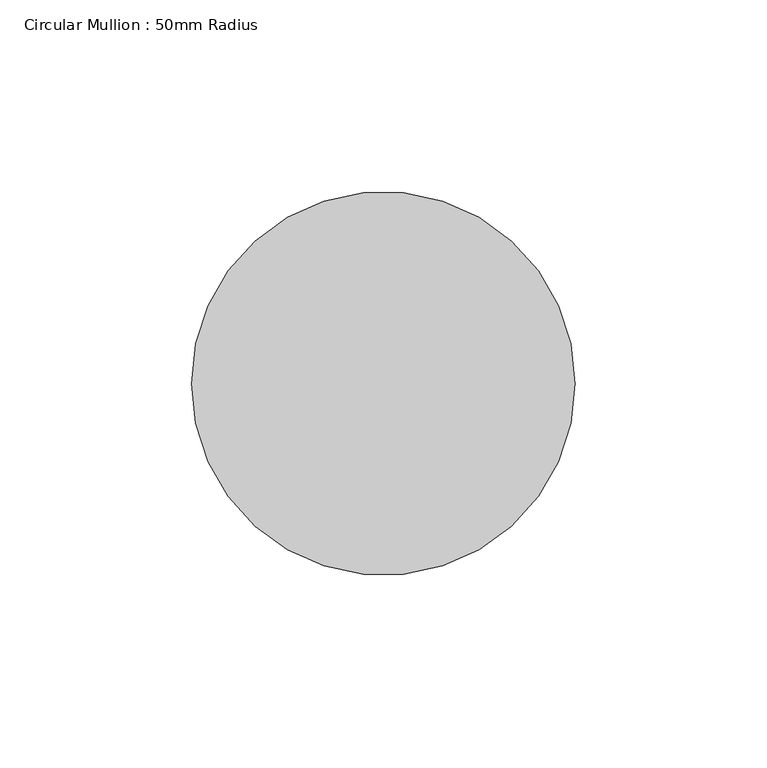
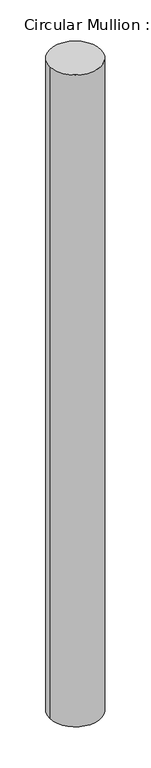
"""IFC4 building model written with IfcOpenShell, lengths in millimetres: member geometry, Circular Mullion : 50mm Radius."""

from ifc_helpers import new_model, si_unit, point, frame, origin, origin_2d, place, context, project, spatial, circle_curve, trimmed, segment, composite_curve, outline, extrude, source, transform, mapped, element, save


def circular_mullion_50mm_radius_13ffe56f(model_context):
    return source(origin(), model_context, "Body", "SweptSolid", [
        extrude(outline(composite_curve([segment(trimmed(circle_curve(origin_2d(), 50.0), [point((50.0, 0.0))], [point((-50.0, 0.0))], False, "CARTESIAN"), True, "CONTINUOUS"), segment(trimmed(circle_curve(origin_2d(), 50.0), [point((-50.0, 0.0))], [point((50.0, 0.0))], False, "CARTESIAN"), True, "CONTINUOUS")], self_intersect=False)), frame((0.0, 0.0, -1346.3366491), z_axis=(0.0, 0.0, 1.0), x_axis=(1.0, 0.0, 0.0)), (0.0, 0.0, 1.0), 1346.3366491),
    ])


if __name__ == "__main__":
    model = new_model("IFC4")
    model_context = context("Model", 3, world=origin())
    ifc_project = project(units=[si_unit("LENGTHUNIT", "METRE", prefix="MILLI")], contexts=[model_context])
    site = spatial("IfcSite", under=ifc_project)
    building = spatial("IfcBuilding", under=site)
    placement = place(None, origin())
    circular_mullion_50mm_radius_shape = circular_mullion_50mm_radius_13ffe56f(model_context)
    element("IfcMember", 1, ObjectType="Circular Mullion : 50mm Radius", at=placement, inside=building, context=model_context, shape_type="MappedRepresentation", body=[
        mapped(circular_mullion_50mm_radius_shape, transform((0.0, 0.0, 0.0), x_axis=(1.0, 0.0, 0.0), y_axis=(0.0, 1.0, 0.0), z_axis=(0.0, 0.0, 1.0))),
    ])
    save(model, "model.ifc")

# Revit data of these elements
# Type "Circular Mullion : 50mm Radius"
#   built-in parameter 1007350 = 0.164042 (stored number, unit not read)
# Element 1 (IfcMember, "Circular Mullion : 50mm Radius")
#   Materials on its faces: "Aluminium"
# Materials
#   "Aluminium": class "Metal", colour RGB 247 247 247, transparency 0, Description = "Aluminium 6061", Cost = 0
